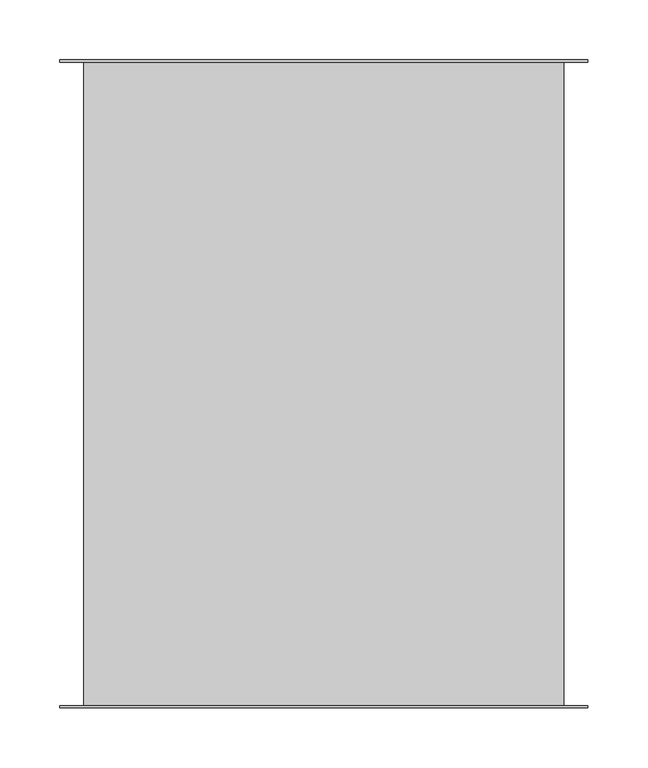
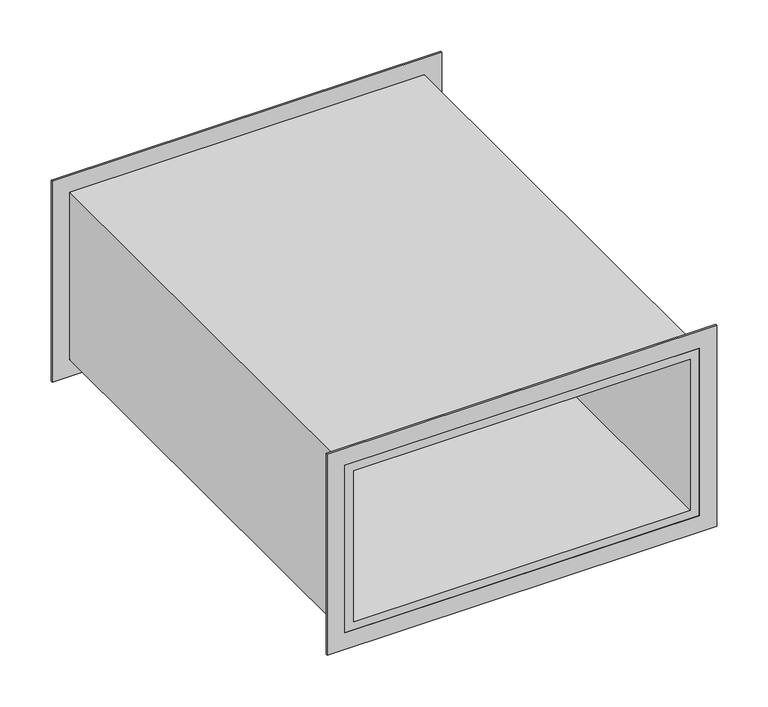
"""IFC4 building model written with IfcOpenShell, lengths in millimetres: proxy geometry, Фильтр карманный DFKR : DFKR 40-20."""

from ifc_helpers import new_model, si_unit, frame, origin, place, context, project, spatial, polyline, outline, extrude, source, transform, mapped, element, save


def mechanical_equipment_d72f12f2(model_context):
    return source(origin(), model_context, "Body", "SweptSolid", [
        extrude(outline(polyline([(120.0, 220.0), (120.0, -220.0), (-120.0, -220.0), (-120.0, 220.0), (120.0, 220.0)]), holes=[polyline([(-100.0, 200.0), (-100.0, -200.0), (100.0, -200.0), (100.0, 200.0), (-100.0, 200.0)])]), frame((0.0, 268.0, 0.0), z_axis=(0.0, 1.0, 0.0), x_axis=(0.0, 0.0, 1.0)), (0.0, 0.0, 1.0), 2.0),
        extrude(outline(polyline([(120.0, -220.0), (-120.0, -220.0), (-120.0, 220.0), (120.0, 220.0), (120.0, -220.0)]), holes=[polyline([(100.0, 200.0), (-100.0, 200.0), (-100.0, -200.0), (100.0, -200.0), (100.0, 200.0)])]), frame((0.0, -270.0, 0.0), z_axis=(0.0, 1.0, 0.0), x_axis=(0.0, 0.0, 1.0)), (0.0, 0.0, 1.0), 2.0),
        extrude(outline(polyline([(100.0, 200.0), (100.0, -200.0), (-100.0, -200.0), (-100.0, 200.0), (100.0, 200.0)]), holes=[polyline([(90.0, 190.0), (-90.0, 190.0), (-90.0, -190.0), (90.0, -190.0), (90.0, 190.0)])]), frame((0.0, -270.0, 0.0), z_axis=(0.0, 1.0, 0.0), x_axis=(0.0, 0.0, 1.0)), (0.0, 0.0, 1.0), 540.0),
    ])


if __name__ == "__main__":
    model = new_model("IFC4")
    model_context = context("Model", 3, world=origin())
    ifc_project = project(units=[si_unit("LENGTHUNIT", "METRE", prefix="MILLI")], contexts=[model_context])
    site = spatial("IfcSite", under=ifc_project)
    building = spatial("IfcBuilding", under=site)
    placement = place(None, origin())
    mechanical_equipment_shape = mechanical_equipment_d72f12f2(model_context)
    element("IfcBuildingElementProxy", 1, Name="Фильтр карманный DFKR : DFKR 40-20", ObjectType="Фильтр карманный DFKR : DFKR 40-20", at=placement, inside=building, context=model_context, shape_type="MappedRepresentation", body=[
        mapped(mechanical_equipment_shape, transform((0.0, 0.0, 0.0), x_axis=(1.0, 0.0, 0.0), y_axis=(0.0, 1.0, 0.0), z_axis=(0.0, 0.0, 1.0))),
    ])
    save(model, "model.ifc")

# Revit data of these elements
# Type "Фильтр карманный DFKR : DFKR 40-20"
#   Manufacturer = "WAER"
#   URL = "https://waer-air.com/"
#   ADSK_Система_Имя [instance default] = ""
#   ADSK_Наименование краткое = "DFKR 40-20"
#   ADSK_Наименование = "Фильтр карманный DFKR 40-20"
#   ADSK_Масса_Текст = "6.5"
#   ADSK_Марка = ""
#   ADSK_Код изделия = ""
#   ADSK_Завод-изготовитель = "WAER"
#   ADSK_Единица измерения = "шт."
#   ADSK_Расход воздуха = 0 m³/h
#   ADSK_Размер_Ширина = 400 mm
#   ADSK_Размер_Длина = 540 mm
#   ADSK_Размер_Высота = 200 mm
#   ADSK_Потеря давления воздуха = 0.0 Pa
#   ADSK_Масса = 6.5
#   ADSK_Количество = 1
#   ADSK_Фильтрующая вставка = element 1329613
#   Default Elevation = 0
#   Keynote = ""
